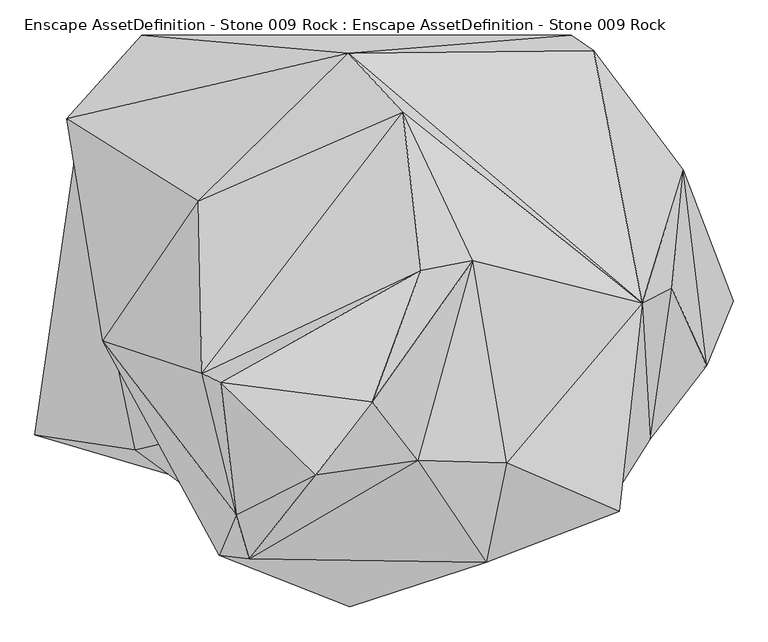
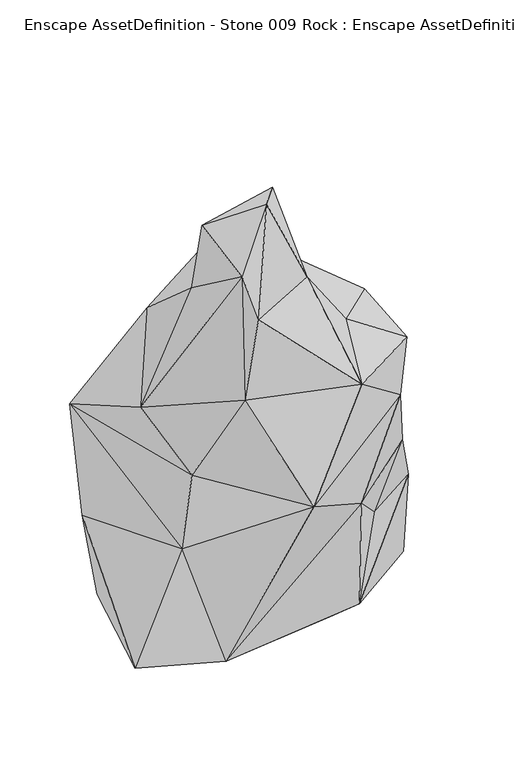
"""IFC4 building model written with IfcOpenShell, lengths in millimetres: geographic element geometry, Enscape AssetDefinition - Stone 009 Rock : Enscape AssetDefinition - Stone 009 Rock."""

from ifc_helpers import new_model, si_unit, origin, place, context, project, spatial, faceted_brep, source, transform, mapped, element, save


def enscape_assetdefinition_stone_009_rock_enscape_b3bb2d2c(model_context):
    return source(origin(), model_context, "Body", "Brep", [
        faceted_brep([(133.1470013, -239.3739969, 1330.597043), (222.1059948, 86.0859975, 1203.5759687), (58.4979989, -144.0339983, 1655.6770802), (498.145014, 17.3959993, 1000.4440546), (108.2609966, 327.7499974, 1162.8530025), (277.3990035, -243.761003, 1116.0999537), (137.8969997, 69.9210018, 1404.6020508), (-33.0369994, -262.7080083, 1692.0170784), (-188.1680042, -112.1710017, 1571.1489916), (-218.8110054, -97.9280025, 1323.9120245), (19.8149998, 424.2910147, 965.5359983), (-224.2009938, 182.791993, 1077.0599842), (-379.8579872, -45.1049991, 873.5209703), (-162.9229933, -328.3970058, 1489.2289639), (-141.6600049, -400.0779986, 1353.8700342), (-189.9310052, -393.8910067, 1046.2239981), (-282.4200094, -211.4859968, 671.2030172), (-438.7840033, 317.6000118, 688.3190274), (-316.1439896, 453.572005, 367.7639961), (-424.3589938, 258.6320043, 276.1569917), (-327.1630108, -222.1679986, 401.9719958), (22.3900005, -477.7970016, 601.2110114), (244.3699986, -405.1100016, 965.7059908), (461.0109925, -322.6070106, 1029.0679932), (434.6860051, -325.25599, 808.382988), (271.4329958, -354.9759984, 453.3709884), (-197.9549974, -283.6380005, -53.5259992), (-490.4209971, -197.8770047, -31.1220009), (305.3910136, -282.0830047, -2.1889999), (250.3429949, -186.2269938, -93.1129977), (-367.9809868, -140.2450055, -76.9419968), (401.5789926, -213.6099935, 287.8130078), (511.334002, -203.9790004, 530.0710201), (646.1669803, 20.7490008, -97.1850008), (603.1489968, -84.8560035, 288.5299921), (-337.2069895, 174.9619991, -119.1409975), (188.9670044, 329.2930126, -92.588), (565.433979, 233.713001, 556.155026), (552.3440242, 214.4159973, 99.8969972), (546.4490056, 41.7860001, 736.9769812), (382.4720085, 453.794986, 477.8980017), (419.1559851, 427.7929962, 703.3280134), (96.1930007, 431.6230118, 23.4779995), (-361.856997, 271.2459862, -67.5119981)], [[[0, 1, 2]], [[1, 3, 4]], [[1, 5, 3]], [[1, 6, 2]], [[1, 0, 5]], [[6, 1, 4]], [[7, 2, 8]], [[2, 6, 8]], [[2, 7, 0]], [[4, 9, 6]], [[8, 6, 9]], [[10, 11, 4]], [[3, 10, 4]], [[9, 4, 11]], [[9, 12, 13]], [[8, 9, 13]], [[9, 11, 12]], [[7, 8, 13]], [[0, 7, 14]], [[14, 7, 13]], [[12, 15, 13]], [[14, 13, 15]], [[16, 12, 17]], [[12, 16, 15]], [[11, 17, 12]], [[11, 10, 17]], [[17, 18, 19]], [[17, 19, 20]], [[20, 16, 17]], [[17, 10, 18]], [[16, 21, 15]], [[21, 16, 20]], [[21, 22, 15]], [[14, 15, 22]], [[22, 0, 14]], [[22, 5, 0]], [[22, 23, 5]], [[21, 24, 22]], [[23, 22, 24]], [[21, 25, 24]], [[21, 20, 26]], [[25, 21, 26]], [[19, 27, 20]], [[27, 26, 20]], [[28, 26, 29]], [[26, 27, 30]], [[26, 28, 25]], [[26, 30, 29]], [[31, 32, 25]], [[31, 25, 28]], [[24, 25, 32]], [[29, 33, 28]], [[34, 28, 33]], [[31, 28, 34]], [[30, 33, 29]], [[30, 27, 35]], [[36, 30, 35]], [[33, 30, 36]], [[37, 33, 38]], [[37, 34, 33]], [[33, 36, 38]], [[34, 37, 39]], [[32, 34, 39]], [[34, 32, 31]], [[39, 37, 3]], [[40, 41, 37]], [[37, 38, 40]], [[37, 41, 3]], [[38, 36, 42]], [[38, 42, 40]], [[36, 43, 42]], [[43, 36, 35]], [[35, 27, 43]], [[19, 18, 43]], [[19, 43, 27]], [[18, 42, 43]], [[40, 42, 18]], [[40, 10, 41]], [[40, 18, 10]], [[10, 3, 41]], [[24, 3, 23]], [[32, 3, 24]], [[32, 39, 3]], [[3, 5, 23]]]),
    ])


if __name__ == "__main__":
    model = new_model("IFC4")
    model_context = context("Model", 3, world=origin())
    ifc_project = project(units=[si_unit("LENGTHUNIT", "METRE", prefix="MILLI")], contexts=[model_context])
    site = spatial("IfcSite", under=ifc_project)
    building = spatial("IfcBuilding", under=site)
    placement = place(None, origin())
    enscape_assetdefinition_stone_009_rock_enscape_shape = enscape_assetdefinition_stone_009_rock_enscape_b3bb2d2c(model_context)
    element("IfcGeographicElement", 1, ObjectType="Enscape AssetDefinition - Stone 009 Rock : Enscape AssetDefinition - Stone 009 Rock", at=placement, inside=building, context=model_context, shape_type="MappedRepresentation", body=[
        mapped(enscape_assetdefinition_stone_009_rock_enscape_shape, transform((0.0, 0.0, 0.0), x_axis=(1.0, 0.0, 0.0), y_axis=(0.0, 1.0, 0.0), z_axis=(0.0, 0.0, 1.0))),
    ])
    save(model, "model.ifc")

# Revit data of these elements
# Type "Enscape AssetDefinition - Stone 009 Rock : Enscape AssetDefinition - Stone 009 Rock"
#   EnscapeAssetSource = "REMOTE"
#   EnscapeAssetId = "b75333a0-b9ae-4542-8500-551a42475bd0"
#   Height = 1.692017 m
#   EnscapeNativeAssetHeight = 1.692017 m
#   Default Elevation = 0
